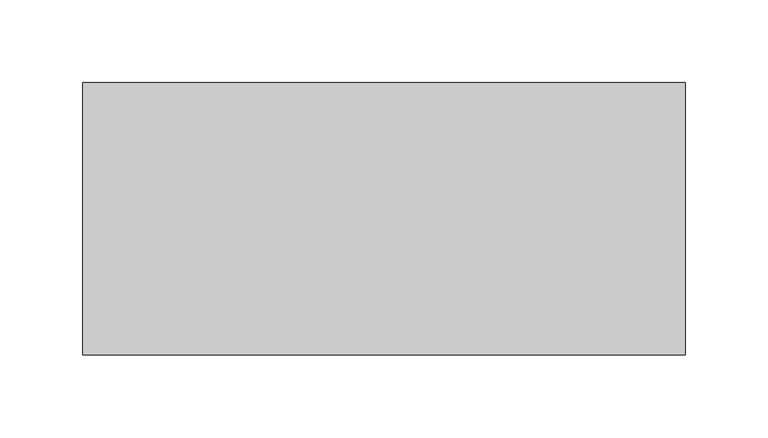
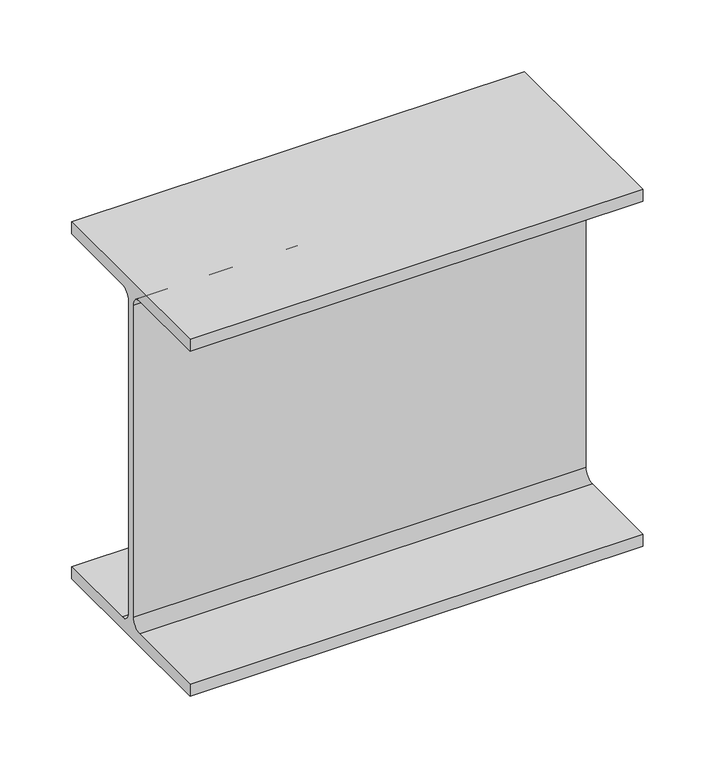
"""IFC4 building model written with IfcOpenShell, lengths in millimetres: beam geometry, Old_Steel Beam_H-KSD3502 : H_SB_ASB_H-300×150x6.5x9."""

from ifc_helpers import new_model, si_unit, point, frame, frame_2d, origin, place, context, project, spatial, polyline, circle_curve, trimmed, segment, composite_curve, outline, extrude, source, transform, mapped, element, save


def beam_05e9ef29(model_context):
    return source(origin(), model_context, "Body", "SweptSolid", [
        extrude(outline(composite_curve([segment(polyline([(82.5, -141.5), (82.5, -151.7), (-82.5, -151.7), (-82.5, -141.5), (-11.9, -141.5)]), True, "CONTINUOUS"), segment(trimmed(circle_curve(frame_2d((-11.9, -132.6)), 8.9), [point((-11.9, -141.5))], [point((-3.0, -132.6))], True, "CARTESIAN"), True, "CONTINUOUS"), segment(polyline([(-3.0, -132.6), (-3.0, 132.6)]), True, "CONTINUOUS"), segment(trimmed(circle_curve(frame_2d((-11.9, 132.6)), 8.9), [point((-3.0, 132.6))], [point((-11.9, 141.5))], True, "CARTESIAN"), True, "CONTINUOUS"), segment(polyline([(-11.9, 141.5), (-82.5, 141.5), (-82.5, 151.7), (82.5, 151.7), (82.5, 141.5), (11.9, 141.5)]), True, "CONTINUOUS"), segment(trimmed(circle_curve(frame_2d((11.9, 132.6)), 8.9), [point((11.9, 141.5))], [point((3.0, 132.6))], True, "CARTESIAN"), True, "CONTINUOUS"), segment(polyline([(3.0, 132.6), (3.0, -132.6)]), True, "CONTINUOUS"), segment(trimmed(circle_curve(frame_2d((11.9, -132.6)), 8.9), [point((3.0, -132.6))], [point((11.9, -141.5))], True, "CARTESIAN"), True, "CONTINUOUS"), segment(polyline([(11.9, -141.5), (82.5, -141.5)]), True, "CONTINUOUS")], self_intersect=False)), frame((-107.3, 0.0, 0.0), z_axis=(1.0, 0.0, 0.0), x_axis=(0.0, 1.0, 0.0)), (0.0, 0.0, 1.0), 364.5999994),
    ])


if __name__ == "__main__":
    model = new_model("IFC4")
    model_context = context("Model", 3, world=origin())
    ifc_project = project(units=[si_unit("LENGTHUNIT", "METRE", prefix="MILLI")], contexts=[model_context])
    site = spatial("IfcSite", under=ifc_project)
    building = spatial("IfcBuilding", under=site)
    placement = place(None, origin())
    beam_shape = beam_05e9ef29(model_context)
    element("IfcBeam", 1, ObjectType="Old_Steel Beam_H-KSD3502 : H_SB_ASB_H-300×150x6.5x9", at=placement, inside=building, context=model_context, shape_type="MappedRepresentation", body=[
        mapped(beam_shape, transform((0.0, 0.0, 0.0), x_axis=(1.0, 0.0, 0.0), y_axis=(0.0, 1.0, 0.0), z_axis=(0.0, 0.0, 1.0))),
    ])
    save(model, "model.ifc")

# Revit data of these elements
# Type "Old_Steel Beam_H-KSD3502 : H_SB_ASB_H-300×150x6.5x9"
#   Width = 15.0 cm
#   Web Thickness = 0.65 cm
#   Web Fillet = 1.3 cm
#   Warping Constant = 107174.0 cm⁶
#   Torsional Moment of Inertia = 9.9539 cm⁴
#   Torsional Modulus = 1.0 cm³
#   Section Area = 46.78 cm²
#   Plastic Modulus weak axis = 105.0 cm³
#   Plastic Modulus strong axis = 542.0 cm³
#   Perimeter = 1.17 m²/m
#   Nominal Weight = 36.70 kgf/m
#   Moment of Inertia weak axis = 508.00 cm⁴
#   Moment of Inertia strong axis = 7210.00 cm⁴
#   Height = 30.0 cm
#   Flange Thickness = 0.9 cm
#   Elastic Modulus weak axis = 67.7 cm³
#   Elastic Modulus strong axis = 481.0 cm³
#   Centroid Vertical = 15.0 cm
#   Centroid Horizontal = 7.5 cm
#   Length [instance default] = 1.5240 m
#   Structural Material [instance default] = Steel, 45-345
#   Assembly Code = ""
# Element 1 (IfcBeam, "Old_Steel Beam_H-KSD3502 : H_SB_ASB_H-300×150x6.5x9")
#   Structural Material = none
# Materials
#   "Steel, 45-345": class "Metal", colour RGB 189 187 185, transparency 0, Description = "Steel 345 MPa", Cost = 0
